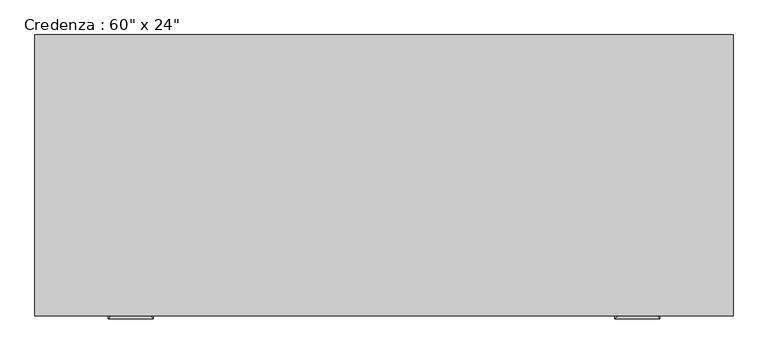
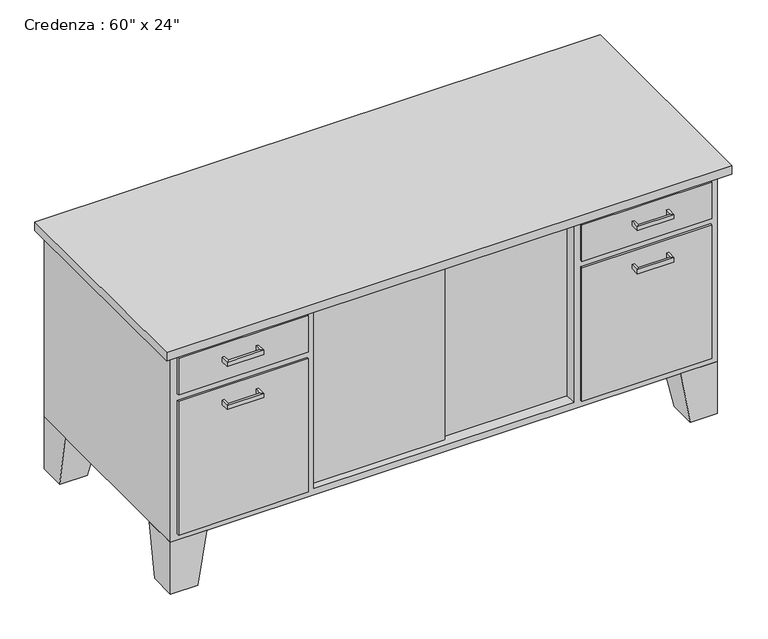
"""IFC4 building model written with IfcOpenShell, lengths in millimetres: furniture geometry."""

from ifc_helpers import new_model, si_unit, frame, origin, place, context, project, spatial, polyline, outline, extrude, faceted_brep, source, transform, mapped, element, save


def furniture_894c625b(model_context):
    return source(origin(), model_context, "Body", "SolidModel", [
        extrude(outline(polyline([(455.5023176, -267.2714583), (46.8442623, -267.2714583), (46.8442623, -254.5714583), (455.5023176, -254.5714583), (455.5023176, -267.2714583)])), frame((0.0, 0.0, 171.45), z_axis=(0.0, 0.0, 1.0), x_axis=(1.0, 0.0, 0.0)), (0.0, 0.0, 1.0), 520.7),
        extrude(outline(polyline([(73.6254475, -279.9714583), (-302.4057377, -279.9714583), (-302.4057377, -267.2714583), (73.6254475, -267.2714583), (73.6254475, -279.9714583)])), frame((0.0, 0.0, 171.45), z_axis=(0.0, 0.0, 1.0), x_axis=(1.0, 0.0, 0.0)), (0.0, 0.0, 1.0), 520.7),
        faceted_brep([(719.9442623, 309.3803279, 152.4), (719.9442623, 207.7803279, 152.4), (821.5442623, 207.7803279, 152.4), (821.5442623, 309.3803279, 152.4), (745.3442623, 309.3803279, 0.0), (821.5442623, 309.3803279, 0.0), (821.5442623, 233.1803279, 0.0), (745.3442623, 233.1803279, 0.0)], [[[0, 1, 2, 3]], [[4, 5, 6, 7]], [[4, 7, 1, 0]], [[7, 6, 2, 1]], [[6, 5, 3, 2]], [[5, 4, 0, 3]]]),
        extrude(outline(polyline([(802.4942623, -306.5696721), (440.5442623, -306.5696721), (440.5442623, -300.2196721), (802.4942623, -300.2196721), (802.4942623, -306.5696721)])), frame((0.0, 0.0, 584.2), z_axis=(0.0, 0.0, 1.0), x_axis=(1.0, 0.0, 0.0)), (0.0, 0.0, 1.0), 107.95),
        extrude(outline(polyline([(802.4942623, -306.5696721), (440.5442623, -306.5696721), (440.5442623, -300.2196721), (802.4942623, -300.2196721), (802.4942623, -306.5696721)])), frame((0.0, 0.0, 171.45), z_axis=(0.0, 0.0, 1.0), x_axis=(1.0, 0.0, 0.0)), (0.0, 0.0, 1.0), 393.7),
        extrude(outline(polyline([(-321.4557377, -306.5696721), (-683.4057377, -306.5696721), (-683.4057377, -300.2196721), (-321.4557377, -300.2196721), (-321.4557377, -306.5696721)])), frame((0.0, 0.0, 584.2), z_axis=(0.0, 0.0, 1.0), x_axis=(1.0, 0.0, 0.0)), (0.0, 0.0, 1.0), 107.95),
        extrude(outline(polyline([(-321.4557377, -306.5696721), (-683.4057377, -306.5696721), (-683.4057377, -300.2196721), (-321.4557377, -300.2196721), (-321.4557377, -306.5696721)])), frame((0.0, 0.0, 171.45), z_axis=(0.0, 0.0, 1.0), x_axis=(1.0, 0.0, 0.0)), (0.0, 0.0, 1.0), 393.7),
        faceted_brep([(-600.8557377, -300.2196721, 152.4), (-600.8557377, -198.6196721, 152.4), (-702.4557377, -198.6196721, 152.4), (-702.4557377, -300.2196721, 152.4), (-626.2557377, -300.2196721, 0.0), (-702.4557377, -300.2196721, 0.0), (-702.4557377, -224.0196721, 0.0), (-626.2557377, -224.0196721, 0.0)], [[[0, 1, 2, 3]], [[4, 5, 6, 7]], [[4, 7, 1, 0]], [[7, 6, 2, 1]], [[6, 5, 3, 2]], [[5, 4, 0, 3]]]),
        faceted_brep([(-600.8557377, 309.3803279, 152.4), (-702.4557377, 309.3803279, 152.4), (-702.4557377, 207.7803279, 152.4), (-600.8557377, 207.7803279, 152.4), (-626.2557377, 309.3803279, 0.0), (-626.2557377, 233.1803279, 0.0), (-702.4557377, 233.1803279, 0.0), (-702.4557377, 309.3803279, 0.0)], [[[0, 1, 2, 3]], [[4, 5, 6, 7]], [[4, 7, 1, 0]], [[7, 6, 2, 1]], [[6, 5, 3, 2]], [[5, 4, 0, 3]]]),
        faceted_brep([(719.9442623, -300.2196721, 152.4), (821.5442623, -300.2196721, 152.4), (821.5442623, -198.6196721, 152.4), (719.9442623, -198.6196721, 152.4), (745.3442623, -300.2196721, 0.0), (745.3442623, -224.0196721, 0.0), (821.5442623, -224.0196721, 0.0), (821.5442623, -300.2196721, 0.0)], [[[0, 1, 2, 3]], [[4, 5, 6, 7]], [[4, 7, 1, 0]], [[7, 6, 2, 1]], [[6, 5, 3, 2]], [[5, 4, 0, 3]]]),
        faceted_brep([(821.5442623, 309.3803279, 711.2), (-702.4557377, 309.3803279, 711.2), (-702.4557377, -300.2196721, 711.2), (821.5442623, -300.2196721, 711.2), (821.5442623, 309.3803279, 152.4), (821.5442623, -300.2196721, 152.4), (-702.4557377, -300.2196721, 152.4), (-702.4557377, 309.3803279, 152.4), (-302.4057377, -300.2196721, 692.15), (421.4942623, -300.2196721, 692.15), (421.4942623, -300.2196721, 171.45), (-302.4057377, -300.2196721, 171.45), (421.4942623, 290.3303279, 692.15), (-302.4057377, 290.3303279, 692.15), (-302.4057377, 290.3303279, 171.45), (421.4942623, 290.3303279, 171.45)], [[[0, 1, 2, 3]], [[4, 5, 6, 7]], [[1, 0, 4, 7]], [[2, 1, 7, 6]], [[3, 2, 6, 5], [8, 9, 10, 11]], [[0, 3, 5, 4]], [[12, 13, 14, 15]], [[13, 12, 9, 8]], [[14, 13, 8, 11]], [[15, 14, 11, 10]], [[12, 15, 10, 9]]]),
        extrude(outline(polyline([(846.9442623, 309.3803279), (846.9442623, -325.6196721), (-727.8557377, -325.6196721), (-727.8557377, 309.3803279), (846.9442623, 309.3803279)])), frame((0.0, 0.0, 711.2), z_axis=(0.0, 0.0, 1.0), x_axis=(1.0, 0.0, 0.0)), (0.0, 0.0, 1.0), 25.4),
        faceted_brep([(-556.4057377, -306.5696721, 527.05), (-556.4057377, -306.5696721, 514.35), (-562.7557377, -306.5696721, 514.35), (-562.7557377, -306.5696721, 527.05), (-556.4057377, -325.6196721, 527.05), (-556.4057377, -325.6196721, 514.35), (-562.7557377, -331.9696721, 514.35), (-562.7557377, -331.9696721, 527.05), (-467.5057377, -325.6196721, 527.05), (-467.5057377, -325.6196721, 514.35), (-461.1557377, -331.9696721, 514.35), (-461.1557377, -331.9696721, 527.05), (-467.5057377, -306.5696721, 527.05), (-461.1557377, -306.5696721, 527.05), (-461.1557377, -306.5696721, 514.35), (-467.5057377, -306.5696721, 514.35)], [[[0, 1, 2, 3]], [[1, 0, 4, 5]], [[2, 1, 5, 6]], [[3, 2, 6, 7]], [[0, 3, 7, 4]], [[5, 4, 8, 9]], [[6, 5, 9, 10]], [[7, 6, 10, 11]], [[4, 7, 11, 8]], [[12, 13, 14, 15]], [[9, 8, 12, 15]], [[10, 9, 15, 14]], [[11, 10, 14, 13]], [[8, 11, 13, 12]]]),
        faceted_brep([(-556.4057377, -306.5696721, 654.05), (-556.4057377, -306.5696721, 641.35), (-562.7557377, -306.5696721, 641.35), (-562.7557377, -306.5696721, 654.05), (-556.4057377, -325.6196721, 654.05), (-556.4057377, -325.6196721, 641.35), (-562.7557377, -331.9696721, 641.35), (-562.7557377, -331.9696721, 654.05), (-467.5057377, -325.6196721, 654.05), (-467.5057377, -325.6196721, 641.35), (-461.1557377, -331.9696721, 641.35), (-461.1557377, -331.9696721, 654.05), (-467.5057377, -306.5696721, 654.05), (-461.1557377, -306.5696721, 654.05), (-461.1557377, -306.5696721, 641.35), (-467.5057377, -306.5696721, 641.35)], [[[0, 1, 2, 3]], [[1, 0, 4, 5]], [[2, 1, 5, 6]], [[3, 2, 6, 7]], [[0, 3, 7, 4]], [[5, 4, 8, 9]], [[6, 5, 9, 10]], [[7, 6, 10, 11]], [[4, 7, 11, 8]], [[12, 13, 14, 15]], [[9, 8, 12, 15]], [[10, 9, 15, 14]], [[11, 10, 14, 13]], [[8, 11, 13, 12]]]),
        faceted_brep([(586.5942623, -306.5696721, 654.1373112), (586.5942623, -306.5696721, 641.4373112), (580.2442623, -306.5696721, 641.4373112), (580.2442623, -306.5696721, 654.1373112), (586.5942623, -325.6196721, 654.1373112), (586.5942623, -325.6196721, 641.4373112), (580.2442623, -331.9696721, 641.4373112), (580.2442623, -331.9696721, 654.1373112), (675.4942623, -325.6196721, 654.1373112), (675.4942623, -325.6196721, 641.4373112), (681.8442623, -331.9696721, 641.4373112), (681.8442623, -331.9696721, 654.1373112), (675.4942623, -306.5696721, 654.1373112), (681.8442623, -306.5696721, 654.1373112), (681.8442623, -306.5696721, 641.4373112), (675.4942623, -306.5696721, 641.4373112)], [[[0, 1, 2, 3]], [[1, 0, 4, 5]], [[2, 1, 5, 6]], [[3, 2, 6, 7]], [[0, 3, 7, 4]], [[5, 4, 8, 9]], [[6, 5, 9, 10]], [[7, 6, 10, 11]], [[4, 7, 11, 8]], [[12, 13, 14, 15]], [[9, 8, 12, 15]], [[10, 9, 15, 14]], [[11, 10, 14, 13]], [[8, 11, 13, 12]]]),
        faceted_brep([(586.5942623, -306.5696721, 527.05), (586.5942623, -306.5696721, 514.35), (580.2442623, -306.5696721, 514.35), (580.2442623, -306.5696721, 527.05), (586.5942623, -325.6196721, 527.05), (586.5942623, -325.6196721, 514.35), (580.2442623, -331.9696721, 514.35), (580.2442623, -331.9696721, 527.05), (675.4942623, -325.6196721, 527.05), (675.4942623, -325.6196721, 514.35), (681.8442623, -331.9696721, 514.35), (681.8442623, -331.9696721, 527.05), (675.4942623, -306.5696721, 527.05), (681.8442623, -306.5696721, 527.05), (681.8442623, -306.5696721, 514.35), (675.4942623, -306.5696721, 514.35)], [[[0, 1, 2, 3]], [[1, 0, 4, 5]], [[2, 1, 5, 6]], [[3, 2, 6, 7]], [[0, 3, 7, 4]], [[5, 4, 8, 9]], [[6, 5, 9, 10]], [[7, 6, 10, 11]], [[4, 7, 11, 8]], [[12, 13, 14, 15]], [[9, 8, 12, 15]], [[10, 9, 15, 14]], [[11, 10, 14, 13]], [[8, 11, 13, 12]]]),
    ])


if __name__ == "__main__":
    model = new_model("IFC4")
    model_context = context("Model", 3, world=origin())
    ifc_project = project(units=[si_unit("LENGTHUNIT", "METRE", prefix="MILLI")], contexts=[model_context])
    site = spatial("IfcSite", under=ifc_project)
    building = spatial("IfcBuilding", under=site)
    placement = place(None, origin())
    furniture_shape = furniture_894c625b(model_context)
    element("IfcFurniture", 1, ObjectType="Credenza : 60\" x 24\"", at=placement, inside=building, context=model_context, shape_type="MappedRepresentation", body=[
        mapped(furniture_shape, transform((0.0, 0.0, 0.0), x_axis=(1.0, 0.0, 0.0), y_axis=(0.0, 1.0, 0.0), z_axis=(0.0, 0.0, 1.0))),
    ])
    save(model, "model.ifc")

# Revit data of these elements
# Type "Credenza : 60\" x 24\""
#   Assembly Code = "E2020200"
#   Depth = 2' - 0"
#   Height = 2' - 5"
#   Width = 5' - 0"
#   Body Material = Laminate, Ivory, Matte
#   Handles/Legs Material = Steel, Chrome Plated
#   Top Material = Cherry
#   Default Elevation = 0
# Element 1 (IfcFurniture, "Credenza : 60\" x 24\"")
#   Materials on its faces: "Steel, Chrome Plated", "Laminate, Ivory, Matte", "Cherry"
# Materials
#   "Laminate, Ivory, Matte": class "Plastic", colour RGB 247 247 239, transparency 0, Description = "Plastic Laminate - Ivory, Matte", Cost = 0
#   "Steel, Chrome Plated": class "Metal", colour RGB 17 17 17, transparency 0, Description = "Chromiuim plated steel", Cost = 0
#   "Cherry": class "Wood", colour RGB 226 177 128, transparency 0, Description = "Prunus Serotina", Cost = 0
